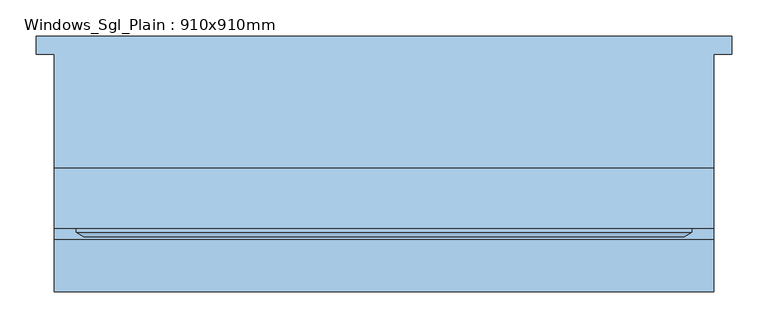
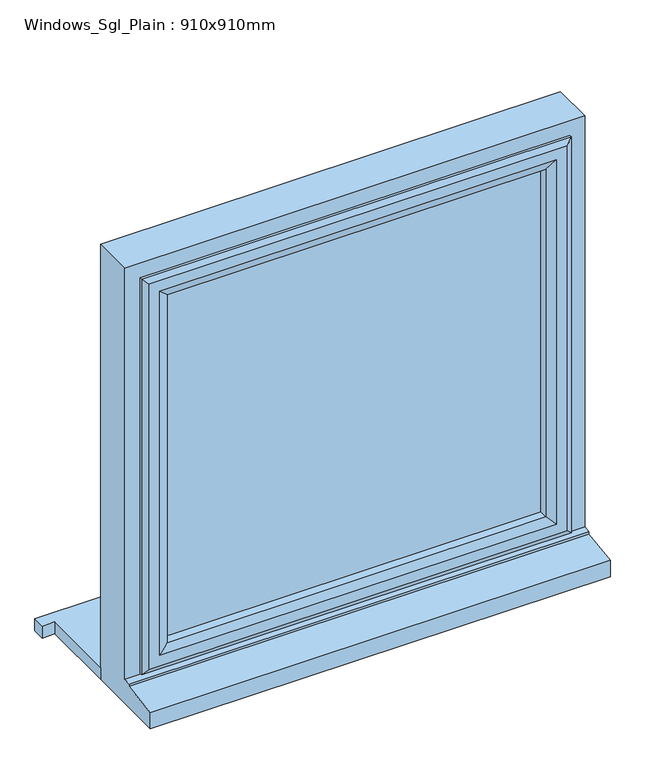
"""IFC4 building model written with IfcOpenShell, lengths in millimetres: window geometry, Windows_Sgl_Plain : 910x910mm."""

from ifc_helpers import new_model, si_unit, frame, origin, place, context, project, spatial, polyline, outline, extrude, faceted_brep, source, transform, mapped, element, save


def windows_sgl_plain_910x910mm_91039d7f(model_context):
    return source(origin(), model_context, "Body", "SolidModel", [
        extrude(outline(polyline([(-480.0, 161.5434322), (480.0, 161.5434322), (480.0, 136.5434322), (455.0, 136.5434322), (455.0, -20.4565678), (-455.0, -20.4565678), (-455.0, 136.5434322), (-480.0, 136.5434322), (-480.0, 161.5434322)])), frame((0.0, 0.0, 1200.0), z_axis=(0.0, 0.0, 1.0), x_axis=(1.0, 0.0, 0.0)), (0.0, 0.0, 1.0), 25.0),
        faceted_brep([(-455.0, -20.4565678, 1200.0), (-455.0, -20.4565678, 2110.0), (455.0, -20.4565678, 2110.0), (455.0, -20.4565678, 1200.0), (-395.0, -20.4565678, 2050.0), (-395.0, -20.4565678, 1275.0), (395.0, -20.4565678, 1275.0), (395.0, -20.4565678, 2050.0), (-455.0, -190.9565678, 1200.0), (-455.0, -190.9565678, 1233.8088847), (-455.0, -118.4565678, 1244.7449676), (-455.0, -118.4565678, 1249.68767), (-455.0, -103.4565678, 1251.0), (-455.0, -103.4565678, 2110.0), (455.0, -103.4565678, 1251.0), (455.0, -103.4565678, 2110.0), (-415.0, -103.4565678, 2070.0), (415.0, -103.4565678, 2070.0), (415.0, -103.4565678, 1263.0), (-415.0, -103.4565678, 1263.0), (-415.0, -38.4565678, 1263.0), (-415.0, -38.4565678, 2070.0), (415.0, -38.4565678, 1263.0), (415.0, -38.4565678, 2070.0), (-395.0, -38.4565678, 2050.0), (395.0, -38.4565678, 2050.0), (395.0, -38.4565678, 1275.0), (-395.0, -38.4565678, 1275.0), (455.0, -118.4565678, 1249.68767), (455.0, -118.4565678, 1244.7449676), (455.0, -190.9565678, 1233.8088847), (455.0, -190.9565678, 1200.0)], [[[0, 1, 2, 3], [4, 5, 6, 7]], [[0, 8, 9, 10, 11, 12, 13, 1]], [[12, 14, 15, 13], [16, 17, 18, 19]], [[19, 20, 21, 16]], [[21, 20, 22, 23], [24, 25, 26, 27]], [[24, 27, 5, 4]], [[1, 13, 15, 2]], [[16, 21, 23, 17]], [[7, 25, 24, 4]], [[14, 28, 29, 30, 31, 3, 2, 15]], [[17, 23, 22, 18]], [[7, 6, 26, 25]], [[31, 8, 0, 3]], [[30, 9, 8, 31]], [[29, 10, 9, 30]], [[28, 11, 10, 29]], [[14, 12, 11, 28]], [[20, 19, 18, 22]], [[5, 27, 26, 6]]]),
        extrude(outline(polyline([(385.0, -67.4565678), (385.0, -91.4565678), (-385.0, -91.4565678), (-385.0, -67.4565678), (385.0, -67.4565678)])), frame((0.0, 0.0, 1293.0), z_axis=(0.0, 0.0, 1.0), x_axis=(1.0, 0.0, 0.0)), (0.0, 0.0, 1.0), 747.0),
        faceted_brep([(-425.0, -103.4565678, 2080.0), (-425.0, -103.4565678, 1253.0), (-425.0, -109.2300705, 1253.0), (-425.0, -109.2300705, 2080.0), (-415.0, -38.4565678, 2070.0), (-415.0, -38.4565678, 1263.0), (-415.0, -103.4565678, 1263.0), (-415.0, -103.4565678, 2070.0), (-375.0, -52.9494677, 2030.0), (-375.0, -52.9494677, 1303.0), (-385.1480377, -38.4565678, 1292.8519623), (-385.1480377, -38.4565678, 2040.1480377), (-375.0, -67.4565678, 2030.0), (-375.0, -67.4565678, 1303.0), (-385.0, -91.4565678, 2040.0), (-385.0, -91.4565678, 1293.0), (-385.0, -67.4565678, 1293.0), (-385.0, -67.4565678, 2040.0), (-375.0, -109.2300705, 2030.0), (-375.0, -109.2300705, 1303.0), (-375.0, -91.4565678, 1303.0), (-375.0, -91.4565678, 2030.0), (-392.4457548, -115.0035732, 2047.4457548), (-392.4457548, -115.0035732, 1285.5542452), (-414.2153903, -115.0035732, 1263.7846097), (-414.2153903, -115.0035732, 2069.2153903), (425.0, -103.4565678, 1253.0), (425.0, -109.2300705, 1253.0), (415.0, -38.4565678, 1263.0), (415.0, -103.4565678, 1263.0), (375.0, -52.9494677, 1303.0), (385.1480377, -38.4565678, 1292.8519623), (375.0, -67.4565678, 1303.0), (385.0, -91.4565678, 1293.0), (385.0, -67.4565678, 1293.0), (375.0, -109.2300705, 1303.0), (375.0, -91.4565678, 1303.0), (392.4457548, -115.0035732, 1285.5542452), (414.2153903, -115.0035732, 1263.7846097), (425.0, -103.4565678, 2080.0), (425.0, -109.2300705, 2080.0), (415.0, -38.4565678, 2070.0), (415.0, -103.4565678, 2070.0), (375.0, -52.9494677, 2030.0), (385.1480377, -38.4565678, 2040.1480377), (375.0, -67.4565678, 2030.0), (385.0, -91.4565678, 2040.0), (385.0, -67.4565678, 2040.0), (375.0, -109.2300705, 2030.0), (375.0, -91.4565678, 2030.0), (392.4457548, -115.0035732, 2047.4457548), (414.2153903, -115.0035732, 2069.2153903)], [[[0, 1, 2, 3]], [[4, 5, 6, 7]], [[8, 9, 10, 11]], [[12, 13, 9, 8]], [[14, 15, 16, 17]], [[18, 19, 20, 21]], [[22, 23, 19, 18]], [[3, 2, 24, 25]], [[1, 26, 27, 2]], [[5, 28, 29, 6]], [[9, 30, 31, 10]], [[13, 32, 30, 9]], [[15, 33, 34, 16]], [[19, 35, 36, 20]], [[23, 37, 35, 19]], [[2, 27, 38, 24]], [[26, 39, 40, 27]], [[28, 41, 42, 29]], [[30, 43, 44, 31]], [[32, 45, 43, 30]], [[33, 46, 47, 34]], [[35, 48, 49, 36]], [[37, 50, 48, 35]], [[27, 40, 51, 38]], [[39, 0, 3, 40]], [[1, 0, 39, 26], [7, 6, 29, 42]], [[41, 4, 7, 42]], [[5, 4, 41, 28], [11, 10, 31, 44]], [[43, 8, 11, 44]], [[45, 12, 8, 43]], [[17, 16, 34, 47], [13, 12, 45, 32]], [[46, 14, 17, 47]], [[15, 14, 46, 33], [21, 20, 36, 49]], [[48, 18, 21, 49]], [[50, 22, 18, 48]], [[25, 24, 38, 51], [23, 22, 50, 37]], [[40, 3, 25, 51]]]),
    ])


if __name__ == "__main__":
    model = new_model("IFC4")
    model_context = context("Model", 3, world=origin())
    ifc_project = project(units=[si_unit("LENGTHUNIT", "METRE", prefix="MILLI")], contexts=[model_context])
    site = spatial("IfcSite", under=ifc_project)
    building = spatial("IfcBuilding", under=site)
    placement = place(None, origin())
    windows_sgl_plain_910x910mm_shape = windows_sgl_plain_910x910mm_91039d7f(model_context)
    element("IfcWindow", 1, ObjectType="Windows_Sgl_Plain : 910x910mm", at=placement, inside=building, context=model_context, shape_type="MappedRepresentation", body=[
        mapped(windows_sgl_plain_910x910mm_shape, transform((0.0, 0.0, 0.0), x_axis=(1.0, 0.0, 0.0), y_axis=(0.0, 1.0, 0.0), z_axis=(0.0, 0.0, 1.0))),
    ])
    save(model, "model.ifc")

# Revit data of these elements
# Type "Windows_Sgl_Plain : 910x910mm"
#   Type Mark = "44"
#   Operation = "SinglePanel"
#   Construction Type Id = "SGL"
#   Manufacturer = "Revit"
#   Keynote = "L10"
#   Analytic Construction = "Large single-glazed windows"
#   Wrap Layers (Ext) from Ext = 102.5 mm
#   Wrap Layers (Int) from Ext = 177.5 mm
#   Window Board Projection = 25 mm
#   Window Board Extension = 25 mm
#   Visual Light Transmittance = 0.9
#   Solar Heat Gain Coefficient = 0.86
#   Rough Width = 910 mm
#   Rough Height = 910 mm
#   Height = 910 mm
#   Width = 910 mm
#   Heat Transfer Coefficient (U) = 5.5617 W/(m²·K)
#   Glazing Thickness = 24 mm
#   FrameOffset - External = 50 mm
#   Frame Depth = 65 mm
#   Default Head Height = 2110 mm
#   Cill Depth = 87.5 mm
#   Cavity Closer Width = 50 mm
#   Cavity Closer Offset from Ext = 102.5 mm
#   Cavity Closer Depth = 85 mm
#   Define Thermal Properties by = 1
#   Vis - Cavity Closers = yes
#   Define Thermal Properties by = 1
#   Material Trim = Window Frame
#   Material Glass = Glass
#   Material Frame = Window Frame
#   Wall Closure = (empty or 0)
# Element 1 (IfcWindow, "Windows_Sgl_Plain : 910x910mm")
#   Materials on its faces: "Window Frame", "Glass"
# Materials
#   "Window Frame": class "Miscellaneous", colour RGB 249 249 249, transparency 0, Keynote = "L10", Cost = 0
#   "Glass": class "Glass", colour RGB 0 128 192, transparency 0.9, Description = "Soda Lime Glass", Cost = 0
